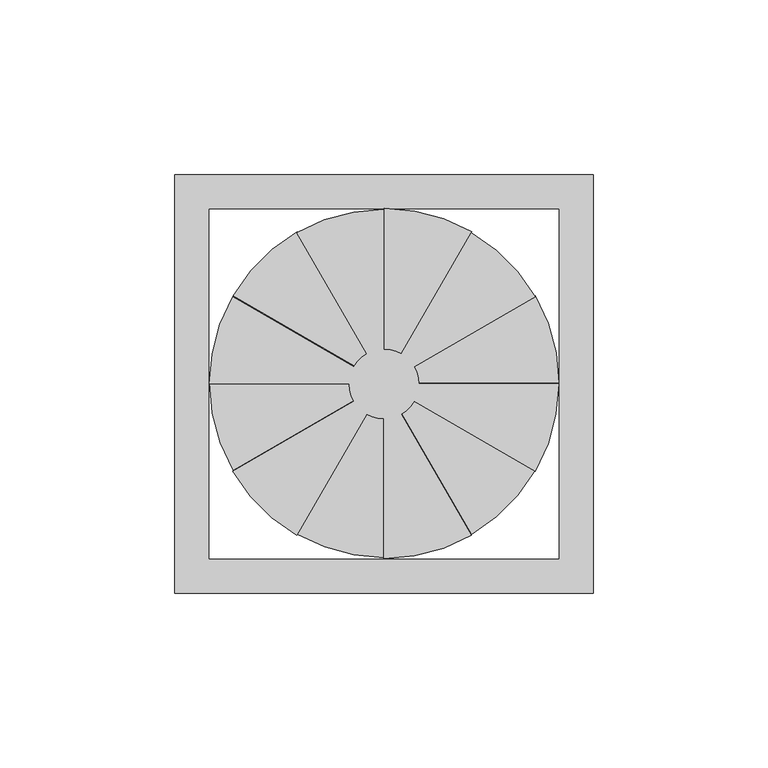
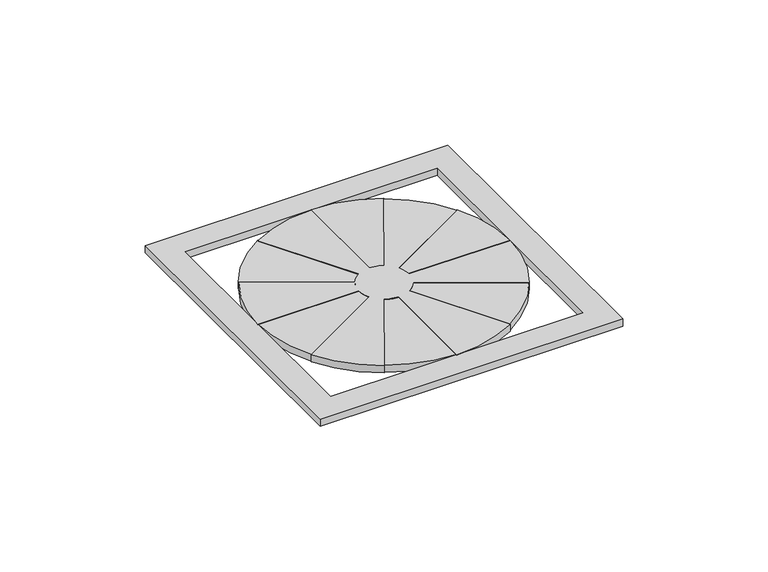
"""IFC4 building model written with IfcOpenShell, lengths in millimetres: proxy geometry, TSP Bathroom Extractor Point-Ceiling : TSP Bathroom Extractor Point-Ceiling."""

from ifc_helpers import new_model, si_unit, point, frame_2d, origin, origin_with_axes, place, context, project, spatial, polyline, circle_curve, trimmed, segment, composite_curve, outline, extrude, source, transform, mapped, element, save


def electrical_fixtures_a255d2e9(model_context):
    return source(origin(), model_context, "Body", "SweptSolid", [
        extrude(outline(composite_curve([segment(trimmed(circle_curve(frame_2d((-50.0, 0.0)), 50.0), [point((-100.0, 0.0))], [point((-93.3012702, 25.0))], False, "CARTESIAN"), True, "CONTINUOUS"), segment(polyline([(-93.3012702, 25.0), (-58.660254, 5.0)]), True, "CONTINUOUS"), segment(trimmed(circle_curve(frame_2d((-50.0, 0.0)), 10.0), [point((-58.660254, 5.0))], [point((-55.0, 8.660254))], False, "CARTESIAN"), True, "CONTINUOUS"), segment(polyline([(-55.0, 8.660254), (-75.0, 43.3012702)]), True, "CONTINUOUS"), segment(trimmed(circle_curve(frame_2d((-50.0, 0.0)), 50.0), [point((-75.0, 43.3012702))], [point((-50.0, 50.0))], False, "CARTESIAN"), True, "CONTINUOUS"), segment(polyline([(-50.0, 50.0), (-50.0, 10.0)]), True, "CONTINUOUS"), segment(trimmed(circle_curve(frame_2d((-50.0, 0.0)), 10.0), [point((-50.0, 10.0))], [point((-45.0, 8.660254))], False, "CARTESIAN"), True, "CONTINUOUS"), segment(polyline([(-45.0, 8.660254), (-25.0, 43.3012702)]), True, "CONTINUOUS"), segment(trimmed(circle_curve(frame_2d((-50.0, 0.0)), 50.0), [point((-25.0, 43.3012702))], [point((-6.6987298, 25.0))], False, "CARTESIAN"), True, "CONTINUOUS"), segment(polyline([(-6.6987298, 25.0), (-41.339746, 5.0)]), True, "CONTINUOUS"), segment(trimmed(circle_curve(frame_2d((-50.0, 0.0)), 10.0), [point((-41.339746, 5.0))], [point((-40.0, 0.0))], False, "CARTESIAN"), True, "CONTINUOUS"), segment(polyline([(-40.0, 0.0), (0.0, 0.0)]), True, "CONTINUOUS"), segment(trimmed(circle_curve(frame_2d((-50.0, 0.0)), 50.0), [point((0.0, 0.0))], [point((-6.6987298, -25.0))], False, "CARTESIAN"), True, "CONTINUOUS"), segment(polyline([(-6.6987298, -25.0), (-41.339746, -5.0)]), True, "CONTINUOUS"), segment(trimmed(circle_curve(frame_2d((-50.0, 0.0)), 10.0), [point((-41.339746, -5.0))], [point((-45.0, -8.660254))], False, "CARTESIAN"), True, "CONTINUOUS"), segment(polyline([(-45.0, -8.660254), (-25.0, -43.3012702)]), True, "CONTINUOUS"), segment(trimmed(circle_curve(frame_2d((-50.0, 0.0)), 50.0), [point((-25.0, -43.3012702))], [point((-50.0, -50.0))], False, "CARTESIAN"), True, "CONTINUOUS"), segment(polyline([(-50.0, -50.0), (-50.0, -10.0)]), True, "CONTINUOUS"), segment(trimmed(circle_curve(frame_2d((-50.0, 0.0)), 10.0), [point((-50.0, -10.0))], [point((-55.0, -8.660254))], False, "CARTESIAN"), True, "CONTINUOUS"), segment(polyline([(-55.0, -8.660254), (-75.0, -43.3012702)]), True, "CONTINUOUS"), segment(trimmed(circle_curve(frame_2d((-50.0, 0.0)), 50.0), [point((-75.0, -43.3012702))], [point((-93.3012702, -25.0))], False, "CARTESIAN"), True, "CONTINUOUS"), segment(polyline([(-93.3012702, -25.0), (-58.660254, -5.0)]), True, "CONTINUOUS"), segment(trimmed(circle_curve(frame_2d((-50.0, 0.0)), 10.0), [point((-58.660254, -5.0))], [point((-60.0, 0.0))], False, "CARTESIAN"), True, "CONTINUOUS"), segment(polyline([(-60.0, 0.0), (-100.0, 0.0)]), True, "CONTINUOUS")], self_intersect=False)), origin_with_axes(), (0.0, 0.0, 1.0), 3.0),
        extrude(outline(composite_curve([segment(trimmed(circle_curve(frame_2d((-49.921082, 0.2945262)), 50.0), [point((-93.2223521, 25.2945262))], [point((-74.921082, 43.5957963))], False, "CARTESIAN"), True, "CONTINUOUS"), segment(polyline([(-74.921082, 43.5957963), (-54.921082, 8.9547802)]), True, "CONTINUOUS"), segment(trimmed(circle_curve(frame_2d((-49.921082, 0.2945262)), 10.0), [point((-54.921082, 8.9547802))], [point((-49.921082, 10.2945262))], False, "CARTESIAN"), True, "CONTINUOUS"), segment(polyline([(-49.921082, 10.2945262), (-49.921082, 50.2945262)]), True, "CONTINUOUS"), segment(trimmed(circle_curve(frame_2d((-49.921082, 0.2945262)), 50.0), [point((-49.921082, 50.2945262))], [point((-24.921082, 43.5957963))], False, "CARTESIAN"), True, "CONTINUOUS"), segment(polyline([(-24.921082, 43.5957963), (-44.921082, 8.9547802)]), True, "CONTINUOUS"), segment(trimmed(circle_curve(frame_2d((-49.921082, 0.2945262)), 10.0), [point((-44.921082, 8.9547802))], [point((-41.2608279, 5.2945262))], False, "CARTESIAN"), True, "CONTINUOUS"), segment(polyline([(-41.2608279, 5.2945262), (-6.6198118, 25.2945262)]), True, "CONTINUOUS"), segment(trimmed(circle_curve(frame_2d((-49.921082, 0.2945262)), 50.0), [point((-6.6198118, 25.2945262))], [point((0.078918, 0.2945262))], False, "CARTESIAN"), True, "CONTINUOUS"), segment(polyline([(0.078918, 0.2945262), (-39.921082, 0.2945262)]), True, "CONTINUOUS"), segment(trimmed(circle_curve(frame_2d((-49.921082, 0.2945262)), 10.0), [point((-39.921082, 0.2945262))], [point((-41.2608279, -4.7054738))], False, "CARTESIAN"), True, "CONTINUOUS"), segment(polyline([(-41.2608279, -4.7054738), (-6.6198118, -24.7054738)]), True, "CONTINUOUS"), segment(trimmed(circle_curve(frame_2d((-49.921082, 0.2945262)), 50.0), [point((-6.6198118, -24.7054738))], [point((-24.921082, -43.006744))], False, "CARTESIAN"), True, "CONTINUOUS"), segment(polyline([(-24.921082, -43.006744), (-44.921082, -8.3657279)]), True, "CONTINUOUS"), segment(trimmed(circle_curve(frame_2d((-49.921082, 0.2945262)), 10.0), [point((-44.921082, -8.3657279))], [point((-49.921082, -9.7054738))], False, "CARTESIAN"), True, "CONTINUOUS"), segment(polyline([(-49.921082, -9.7054738), (-49.921082, -49.7054738)]), True, "CONTINUOUS"), segment(trimmed(circle_curve(frame_2d((-49.921082, 0.2945262)), 50.0), [point((-49.921082, -49.7054738))], [point((-74.921082, -43.006744))], False, "CARTESIAN"), True, "CONTINUOUS"), segment(polyline([(-74.921082, -43.006744), (-54.921082, -8.3657279)]), True, "CONTINUOUS"), segment(trimmed(circle_curve(frame_2d((-49.921082, 0.2945262)), 10.0), [point((-54.921082, -8.3657279))], [point((-58.581336, -4.7054738))], False, "CARTESIAN"), True, "CONTINUOUS"), segment(polyline([(-58.581336, -4.7054738), (-93.2223521, -24.7054738)]), True, "CONTINUOUS"), segment(trimmed(circle_curve(frame_2d((-49.921082, 0.2945262)), 50.0), [point((-93.2223521, -24.7054738))], [point((-99.921082, 0.2945262))], False, "CARTESIAN"), True, "CONTINUOUS"), segment(polyline([(-99.921082, 0.2945262), (-59.921082, 0.2945262)]), True, "CONTINUOUS"), segment(trimmed(circle_curve(frame_2d((-49.921082, 0.2945262)), 10.0), [point((-59.921082, 0.2945262))], [point((-58.581336, 5.2945262))], False, "CARTESIAN"), True, "CONTINUOUS"), segment(polyline([(-58.581336, 5.2945262), (-93.2223521, 25.2945262)]), True, "CONTINUOUS")], self_intersect=False)), origin_with_axes(), (0.0, 0.0, 1.0), 3.0),
        extrude(outline(polyline([(10.0, 60.0), (10.0, -60.0), (-110.0, -60.0), (-110.0, 60.0), (10.0, 60.0)]), holes=[polyline([(-100.0, 50.0), (-100.0, -50.0), (0.0, -50.0), (0.0, 50.0), (-100.0, 50.0)])]), origin_with_axes(), (0.0, 0.0, 1.0), 3.0),
    ])


if __name__ == "__main__":
    model = new_model("IFC4")
    model_context = context("Model", 3, world=origin())
    ifc_project = project(units=[si_unit("LENGTHUNIT", "METRE", prefix="MILLI")], contexts=[model_context])
    site = spatial("IfcSite", under=ifc_project)
    building = spatial("IfcBuilding", under=site)
    placement = place(None, origin())
    electrical_fixtures_shape = electrical_fixtures_a255d2e9(model_context)
    element("IfcBuildingElementProxy", 1, Name="TSP Bathroom Extractor Point-Ceiling : TSP Bathroom Extractor Point-Ceiling", ObjectType="TSP Bathroom Extractor Point-Ceiling : TSP Bathroom Extractor Point-Ceiling", at=placement, inside=building, context=model_context, shape_type="MappedRepresentation", body=[
        mapped(electrical_fixtures_shape, transform((0.0, 0.0, 0.0), x_axis=(1.0, 0.0, 0.0), y_axis=(0.0, 1.0, 0.0), z_axis=(0.0, 0.0, 1.0))),
    ])
    save(model, "model.ifc")

# Revit data of these elements
# Type "TSP Bathroom Extractor Point-Ceiling : TSP Bathroom Extractor Point-Ceiling"
#   Model = "TSP_ELECBEFPC"
#   Default Elevation = 0
# Element 1 (IfcBuildingElementProxy, "TSP Bathroom Extractor Point-Ceiling : TSP Bathroom Extractor Point-Ceiling")
#   Materials on its faces: "Plastic, Opaque Black", "Aluminum, Anodized Blue"
# Materials
#   "Plastic, Opaque Black": class "Plastic", colour RGB 0 0 0, transparency 0.7, Description = "Plastic, generic, opaque black", Cost = 0
#   "Aluminum, Anodized Blue": class "Metal", colour RGB 120 120 120, transparency 0, Description = "Anodized aluminum, blue", Cost = 0
